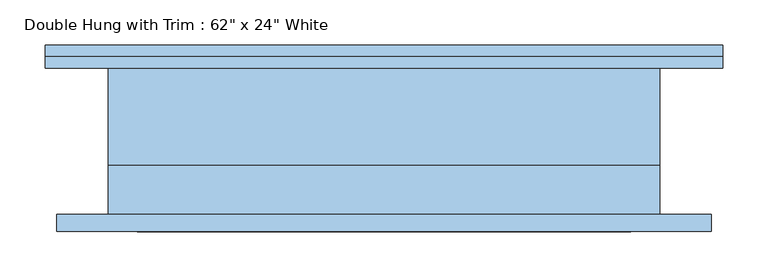
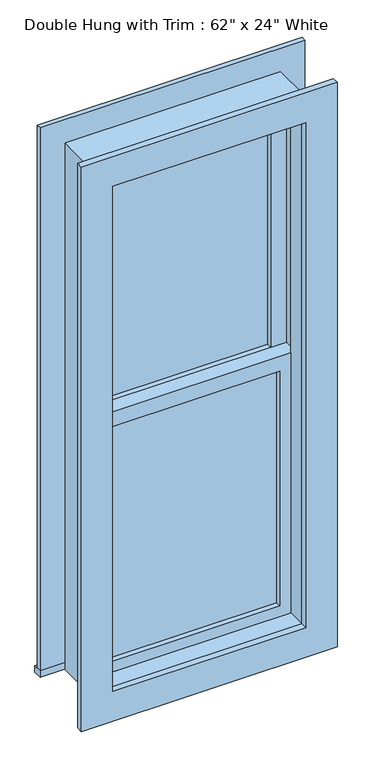
"""IFC4 building model written with IfcOpenShell, lengths in millimetres: window geometry."""

from ifc_helpers import new_model, si_unit, frame, origin, place, context, project, spatial, polyline, outline, extrude, source, transform, mapped, element, save


def window_3658052a(model_context):
    return source(origin(), model_context, "Body", "SweptSolid", [
        extrude(outline(polyline([(-241.3, 1.5875), (241.3, 1.5875), (241.3, -11.1125), (-241.3, -11.1125), (-241.3, 1.5875)])), frame((0.0, 0.0, 977.9), z_axis=(0.0, 0.0, 1.0), x_axis=(1.0, 0.0, 0.0)), (0.0, 0.0, 1.0), 701.675),
        extrude(outline(polyline([(1724.025, -285.75), (933.45, -285.75), (933.45, 285.75), (1724.025, 285.75), (1724.025, -285.75)]), holes=[polyline([(1679.575, -241.3), (1679.575, 241.3), (977.9, 241.3), (977.9, -241.3), (1679.575, -241.3)])]), frame((0.0, -26.9875, 0.0), z_axis=(0.0, 1.0, 0.0), x_axis=(0.0, 0.0, 1.0)), (0.0, 0.0, 1.0), 44.45),
        extrude(outline(polyline([(-374.65, 106.3625), (374.65, 106.3625), (374.65, 80.9625), (-374.65, 80.9625), (-374.65, 106.3625)])), frame((0.0, 0.0, 914.4), z_axis=(0.0, 0.0, 1.0), x_axis=(1.0, 0.0, 0.0)), (0.0, 0.0, 1.0), 19.05),
        extrude(outline(polyline([(2470.15, -285.75), (2470.15, 285.75), (933.45, 285.75), (933.45, 374.65), (2559.05, 374.65), (2559.05, -374.65), (933.45, -374.65), (933.45, -285.75), (2470.15, -285.75)])), frame((0.0, 80.9625, 0.0), z_axis=(0.0, 1.0, 0.0), x_axis=(0.0, 0.0, 1.0)), (0.0, 0.0, 1.0), 12.7),
        extrude(outline(polyline([(2546.35, 361.95), (2546.35, -361.95), (857.25, -361.95), (857.25, 361.95), (2546.35, 361.95)]), holes=[polyline([(2457.45, 273.05), (946.15, 273.05), (946.15, -273.05), (2457.45, -273.05), (2457.45, 273.05)])]), frame((0.0, -100.0125, 0.0), z_axis=(0.0, 1.0, 0.0), x_axis=(0.0, 0.0, 1.0)), (0.0, 0.0, 1.0), 19.05),
        extrude(outline(polyline([(241.3, 33.3375), (-241.3, 33.3375), (-241.3, 46.0375), (241.3, 46.0375), (241.3, 33.3375)])), frame((0.0, 0.0, 1724.025), z_axis=(0.0, 0.0, 1.0), x_axis=(1.0, 0.0, 0.0)), (0.0, 0.0, 1.0), 701.675),
        extrude(outline(polyline([(2470.15, -285.75), (1679.575, -285.75), (1679.575, 285.75), (2470.15, 285.75), (2470.15, -285.75)]), holes=[polyline([(2425.7, -241.3), (2425.7, 241.3), (1724.025, 241.3), (1724.025, -241.3), (2425.7, -241.3)])]), frame((0.0, 17.4625, 0.0), z_axis=(0.0, 1.0, 0.0), x_axis=(0.0, 0.0, 1.0)), (0.0, 0.0, 1.0), 44.45),
        extrude(outline(polyline([(2489.2, -304.8), (914.4, -304.8), (914.4, 304.8), (2489.2, 304.8), (2489.2, -304.8)]), holes=[polyline([(2457.45, -273.05), (2457.45, 273.05), (946.15, 273.05), (946.15, -273.05), (2457.45, -273.05)])]), frame((0.0, -80.9625, 0.0), z_axis=(0.0, 1.0, 0.0), x_axis=(0.0, 0.0, 1.0)), (0.0, 0.0, 1.0), 53.975),
        extrude(outline(polyline([(2489.2, 304.8), (2489.2, -304.8), (914.4, -304.8), (914.4, 304.8), (2489.2, 304.8)]), holes=[polyline([(2470.15, 285.75), (933.45, 285.75), (933.45, -285.75), (2470.15, -285.75), (2470.15, 285.75)])]), frame((0.0, -26.9875, 0.0), z_axis=(0.0, 1.0, 0.0), x_axis=(0.0, 0.0, 1.0)), (0.0, 0.0, 1.0), 107.95),
    ])


if __name__ == "__main__":
    model = new_model("IFC4")
    model_context = context("Model", 3, world=origin())
    ifc_project = project(units=[si_unit("LENGTHUNIT", "METRE", prefix="MILLI")], contexts=[model_context])
    site = spatial("IfcSite", under=ifc_project)
    building = spatial("IfcBuilding", under=site)
    placement = place(None, origin())
    window_shape = window_3658052a(model_context)
    element("IfcWindow", 1, ObjectType="Double Hung with Trim : 62\" x 24\" White", at=placement, inside=building, context=model_context, shape_type="MappedRepresentation", body=[
        mapped(window_shape, transform((0.0, 0.0, 0.0), x_axis=(1.0, 0.0, 0.0), y_axis=(0.0, 1.0, 0.0), z_axis=(0.0, 0.0, 1.0))),
    ])
    save(model, "model.ifc")

# Revit data of these elements
# Type "Double Hung with Trim : 62\" x 24\" White"
#   Type Mark = "77"
#   Construction Type Id = "GSP4R"
#   Assembly Code = "B2020100"
#   Analytic Construction = "1/8 in Pilkington single glazing"
#   Visual Light Transmittance = 0.9
#   Solar Heat Gain Coefficient = 0.78
#   Heat Transfer Coefficient (U) = 3.6886 W/(m²·K)
#   Height = 5' - 2"
#   Default Sill Height = 3' - 0"
#   Trim Projection - Ext. = 0' - 0 1/2"
#   Trim Projection - Int. = 0' - 0 3/4"
#   Trim Width - Exterior = 0' - 3 1/2"
#   Trim Width - Interior = 0' - 3 1/2"
#   Width = 2' - 0"
#   Window Inset = 0' - 0 3/4"
#   COBie.Type = no
#   Glass Pane Material = Glass
#   Sash Material = Sash - White
#   Trim Exterior Material = Trim - White
#   Trim Interior Material = Trim - White
#   Wall Closure = (empty or 0)
# Element 1 (IfcWindow, "Double Hung with Trim : 62\" x 24\" White")
#   Materials on its faces: "Sash - White", "Trim - White", "Glass"
# Materials
#   "Glass": class "Glass", colour RGB 0 128 192, transparency 0.75, Description = "Soda Lime Glass", Cost = 0
#   "Sash - White": class "Wood", colour RGB 255 255 255, transparency 0, Cost = 0
#   "Trim - White": class "Wood", colour RGB 255 255 255, transparency 0, Cost = 0
